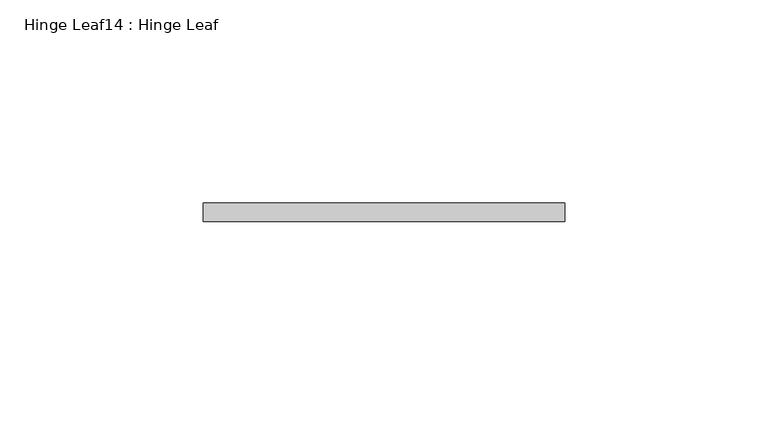
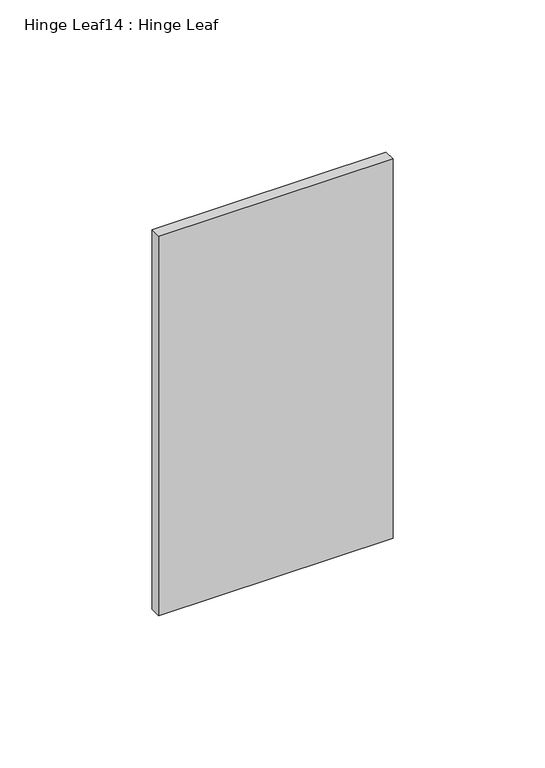
"""IFC4 building model written with IfcOpenShell, lengths in millimetres: proxy geometry, Hinge Leaf14 : Hinge Leaf."""

from ifc_helpers import new_model, si_unit, frame, origin, place, context, project, spatial, polyline, outline, extrude, source, transform, mapped, element, save


def hinge_leaf14_hinge_leaf_d7f0489c(model_context):
    return source(origin(), model_context, "Body", "SweptSolid", [
        extrude(outline(polyline([(587327.7934739, -534104.7943841), (587416.6934739, -534104.7943841), (587416.6934739, -534109.3663841), (587327.7934739, -534109.3663841), (587327.7934739, -534104.7943841)])), frame((0.0, 0.0, 311.15), z_axis=(0.0, 0.0, 1.0), x_axis=(1.0, 0.0, 0.0)), (0.0, 0.0, 1.0), 152.4),
    ])


if __name__ == "__main__":
    model = new_model("IFC4")
    model_context = context("Model", 3, world=origin())
    ifc_project = project(units=[si_unit("LENGTHUNIT", "METRE", prefix="MILLI")], contexts=[model_context])
    site = spatial("IfcSite", under=ifc_project)
    building = spatial("IfcBuilding", under=site)
    placement = place(None, origin())
    hinge_leaf14_hinge_leaf_shape = hinge_leaf14_hinge_leaf_d7f0489c(model_context)
    element("IfcBuildingElementProxy", 1, Name="Hinge Leaf14 : Hinge Leaf", ObjectType="Hinge Leaf14 : Hinge Leaf", at=placement, inside=building, context=model_context, shape_type="MappedRepresentation", body=[
        mapped(hinge_leaf14_hinge_leaf_shape, transform((0.0, 0.0, 0.0), x_axis=(1.0, 0.0, 0.0), y_axis=(0.0, 1.0, 0.0), z_axis=(0.0, 0.0, 1.0))),
    ])
    save(model, "model.ifc")

# Revit data of these elements
# Element 1 (IfcBuildingElementProxy, "Hinge Leaf14 : Hinge Leaf")
#   Materials on its faces: "6\"X6\" WELD-ON STL BUTT HINGE"
# Materials
#   "6\"X6\" WELD-ON STL BUTT HINGE": class "Metal", colour RGB 189 187 185, transparency 0, Description = "Carbon steel", Cost = 0
